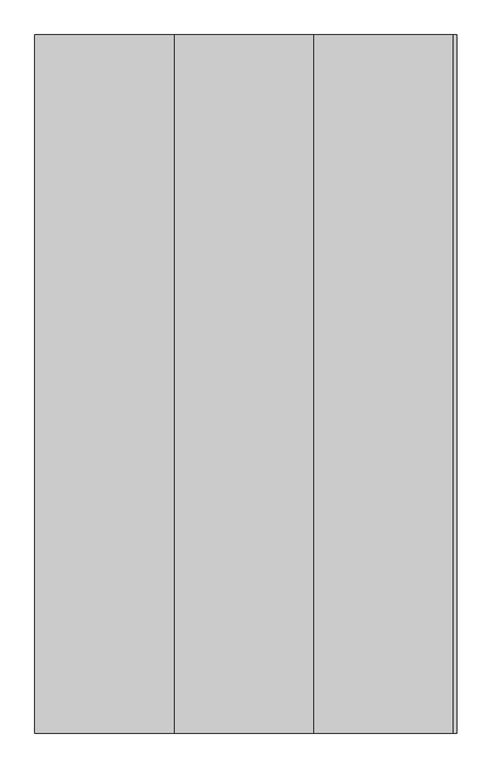
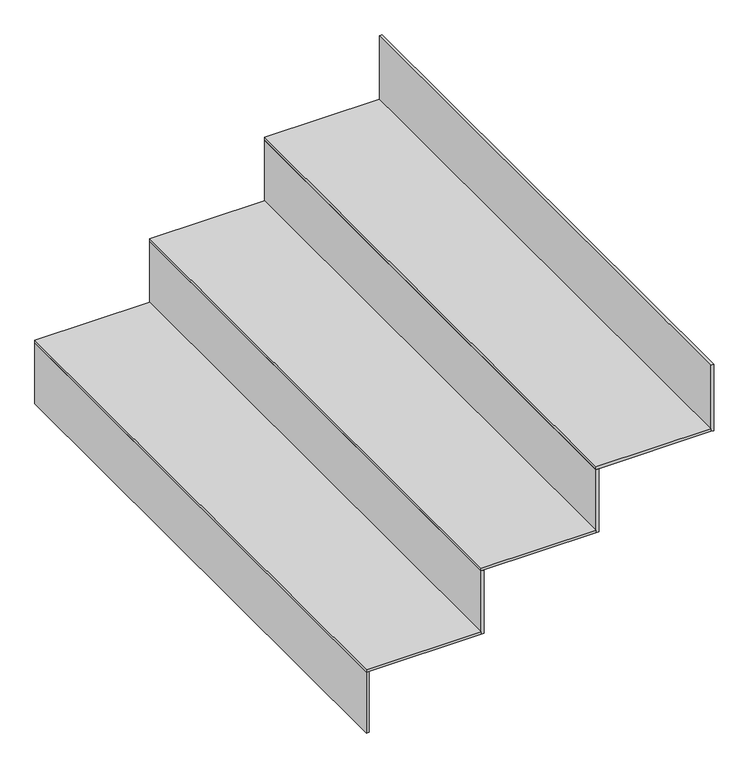
"""IFC4 building model written with IfcOpenShell, lengths in millimetres: stair flight geometry."""

from ifc_helpers import new_model, si_unit, frame, origin, place, context, project, spatial, polyline, outline, extrude, source, transform, mapped, element, save


def stair_flight_0d36ccc0(model_context):
    return source(origin(), model_context, "Body", "SweptSolid", [
        extrude(outline(polyline([(51850.0, -8350.0), (51850.0, -9850.0), (51550.0, -9850.0), (51550.0, -8350.0), (51850.0, -8350.0)])), frame((0.0, 0.0, 14267.5), z_axis=(0.0, 0.0, 1.0), x_axis=(1.0, 0.0, 0.0)), (0.0, 0.0, 1.0), 7.5),
        extrude(outline(polyline([(52150.0, -8350.0), (52150.0, -9850.0), (51850.0, -9850.0), (51850.0, -8350.0), (52150.0, -8350.0)])), frame((0.0, 0.0, 14442.5), z_axis=(0.0, 0.0, 1.0), x_axis=(1.0, 0.0, 0.0)), (0.0, 0.0, 1.0), 7.5),
        extrude(outline(polyline([(52450.0, -8350.0), (52450.0, -9850.0), (52150.0, -9850.0), (52150.0, -8350.0), (52450.0, -8350.0)])), frame((0.0, 0.0, 14617.5), z_axis=(0.0, 0.0, 1.0), x_axis=(1.0, 0.0, 0.0)), (0.0, 0.0, 1.0), 7.5),
        extrude(outline(polyline([(51557.5, -9850.0), (51550.0, -9850.0), (51550.0, -8350.0), (51557.5, -8350.0), (51557.5, -9850.0)])), frame((0.0, 0.0, 14100.0), z_axis=(0.0, 0.0, 1.0), x_axis=(1.0, 0.0, 0.0)), (0.0, 0.0, 1.0), 167.5),
        extrude(outline(polyline([(51857.5, -9850.0), (51850.0, -9850.0), (51850.0, -8350.0), (51857.5, -8350.0), (51857.5, -9850.0)])), frame((0.0, 0.0, 14267.5), z_axis=(0.0, 0.0, 1.0), x_axis=(1.0, 0.0, 0.0)), (0.0, 0.0, 1.0), 175.0),
        extrude(outline(polyline([(52157.5, -9850.0), (52150.0, -9850.0), (52150.0, -8350.0), (52157.5, -8350.0), (52157.5, -9850.0)])), frame((0.0, 0.0, 14442.5), z_axis=(0.0, 0.0, 1.0), x_axis=(1.0, 0.0, 0.0)), (0.0, 0.0, 1.0), 175.0),
        extrude(outline(polyline([(52457.5, -9850.0), (52450.0, -9850.0), (52450.0, -8350.0), (52457.5, -8350.0), (52457.5, -9850.0)])), frame((0.0, 0.0, 14617.5), z_axis=(0.0, 0.0, 1.0), x_axis=(1.0, 0.0, 0.0)), (0.0, 0.0, 1.0), 182.5),
    ])


if __name__ == "__main__":
    model = new_model("IFC4")
    model_context = context("Model", 3, world=origin())
    ifc_project = project(units=[si_unit("LENGTHUNIT", "METRE", prefix="MILLI")], contexts=[model_context])
    site = spatial("IfcSite", under=ifc_project)
    building = spatial("IfcBuilding", under=site)
    placement = place(None, origin())
    stair_flight_shape = stair_flight_0d36ccc0(model_context)
    element("IfcStairFlight", 1, at=placement, inside=building, context=model_context, shape_type="MappedRepresentation", body=[
        mapped(stair_flight_shape, transform((0.0, 0.0, 0.0), x_axis=(1.0, 0.0, 0.0), y_axis=(0.0, 1.0, 0.0), z_axis=(0.0, 0.0, 1.0))),
    ])
    save(model, "model.ifc")

# Revit data of these elements
# Element 1 (IfcStairFlight)
#   Materials on its faces: "00_Finish_Conduction Tile"
# Materials
#   "00_Finish_Conduction Tile": class "Finish", colour RGB 245 245 245, transparency 0, Description = "Ceramic Tile", Cost = 0
